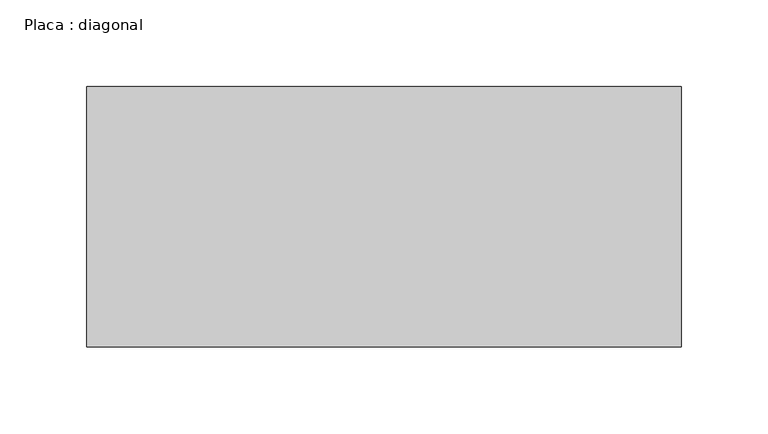
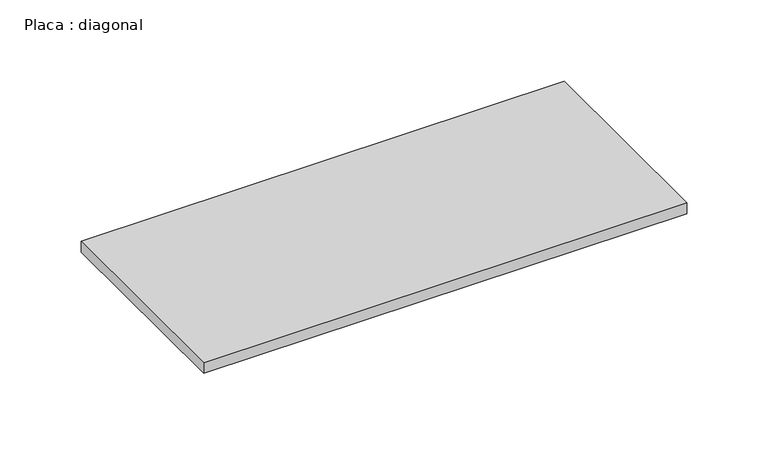
"""IFC4 building model written with IfcOpenShell, lengths in millimetres: beam geometry, Placa : diagonal."""

from ifc_helpers import new_model, si_unit, frame, origin, place, context, project, spatial, polyline, outline, extrude, source, transform, mapped, element, save


def placa_diagonal_c2f8bddd(model_context):
    return source(origin(), model_context, "Body", "SweptSolid", [
        extrude(outline(polyline([(170.6977754, 75.0), (170.6977754, -75.0), (-171.6122385, -75.0), (-171.6122385, 75.0), (170.6977754, 75.0)])), frame((0.0, 0.0, -4.0), z_axis=(0.0, 0.0, 1.0), x_axis=(1.0, 0.0, 0.0)), (0.0, 0.0, 1.0), 8.0),
    ])


if __name__ == "__main__":
    model = new_model("IFC4")
    model_context = context("Model", 3, world=origin())
    ifc_project = project(units=[si_unit("LENGTHUNIT", "METRE", prefix="MILLI")], contexts=[model_context])
    site = spatial("IfcSite", under=ifc_project)
    building = spatial("IfcBuilding", under=site)
    placement = place(None, origin())
    placa_diagonal_shape = placa_diagonal_c2f8bddd(model_context)
    element("IfcBeam", 1, ObjectType="Placa : diagonal", at=placement, inside=building, context=model_context, shape_type="MappedRepresentation", body=[
        mapped(placa_diagonal_shape, transform((0.0, 0.0, 0.0), x_axis=(1.0, 0.0, 0.0), y_axis=(0.0, 1.0, 0.0), z_axis=(0.0, 0.0, 1.0))),
    ])
    save(model, "model.ifc")

# Revit data of these elements
# Type "Placa : diagonal"
#   W = 0
#   Length [instance default] = 1.50 m
#   b = 0.15 m
#   d = 0.008 m
#   A = 0 m²
#   Structural Material [instance default] = Aço, 45-345
# Element 1 (IfcBeam, "Placa : diagonal")
#   Materials on its faces: "Aço, 45-345"
# Materials
#   "Aço, 45-345": class "Metal", colour RGB 247 247 247, transparency 0, Description = "Aço 345 MPa", Cost = 0
